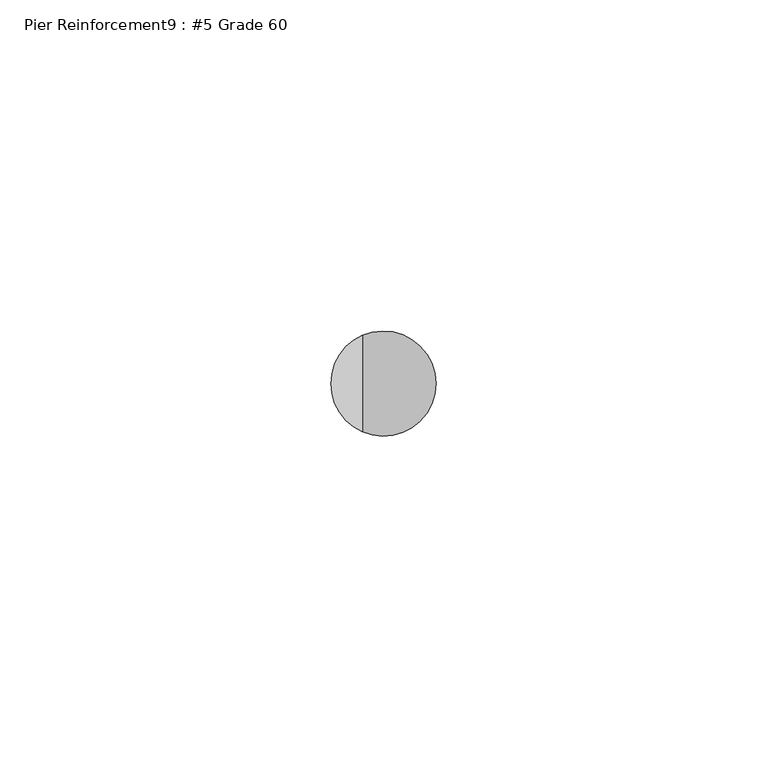
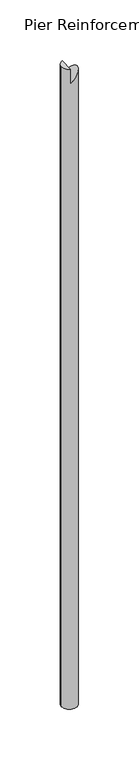
"""IFC4 building model written with IfcOpenShell, lengths in millimetres: proxy geometry, Pier Reinforcement9 : #5 Grade 60."""

from ifc_helpers import new_model, si_unit, frame, origin, place, context, project, spatial, circle_curve, ellipse_curve, source, transform, mapped, element, save
from ifc_brep_helpers import plane_surface, cylinder_surface, advanced_brep


def pier_reinforcement9_5_grade_60_f625620a(model_context):
    return source(origin(), model_context, "Body", "AdvancedBrep", [
        advanced_brep(
        [(590218.1172365, -534096.6663841, -47.625), (590222.8797365, -534103.941223, -47.625), (590222.8797365, -534089.3915452, -47.625), (590218.1172365, -534096.6663841, -733.425), (590233.9922365, -534096.6663841, -733.425), (590233.9922365, -534096.6663841, -52.3875), (590222.8797365, -534103.941223, -63.5), (590222.8797365, -534089.3915452, -63.5)],
        [
            (0, 1, circle_curve(frame((590226.0547365, -534096.6663841, -47.625), z_axis=(0.0, 0.0, 1.0), x_axis=(1.0, 0.0, 0.0)), 7.9375)),
            (1, 2),
            (2, 0, circle_curve(frame((590226.0547365, -534096.6663841, -47.625), z_axis=(0.0, 0.0, 1.0), x_axis=(1.0, 0.0, 0.0)), 7.9375)),
            (3, 4, circle_curve(frame((590226.0547365, -534096.6663841, -733.425), z_axis=(0.0, 0.0, -1.0), x_axis=(1.0, 0.0, 0.0)), 7.9375)),
            (4, 3, circle_curve(frame((590226.0547365, -534096.6663841, -733.425), z_axis=(0.0, 0.0, -1.0), x_axis=(1.0, 0.0, 0.0)), 7.9375)),
            (4, 5),
            (5, 6, ellipse_curve(frame((590226.0547365, -534096.6663841, -60.325), z_axis=(0.707106781186547, 0.0, -0.7071067811865481), x_axis=(0.7071067811865481, 0.0, 0.7071067811865468)), 11.2253202, 7.9375)),
            (6, 1),
            (0, 3),
            (2, 7),
            (7, 5, ellipse_curve(frame((590226.0547365, -534096.6663841, -60.325), z_axis=(0.707106781186547, 0.0, -0.7071067811865481), x_axis=(0.7071067811865481, 0.0, 0.7071067811865468)), 11.2253202, 7.9375)),
            (6, 7),
        ],
        [
            plane_surface(frame((590233.9922365, -534096.6663841, -47.625), z_axis=(0.0, 0.0, 1.0), x_axis=(0.0, 1.0, 0.0))),
            plane_surface(frame((590233.9922365, -534096.6663841, -733.425), z_axis=(0.0, 0.0, -1.0), x_axis=(0.0, -1.0, 0.0))),
            cylinder_surface(frame((590226.0547365, -534096.6663841, -733.425), z_axis=(0.0, 0.0, 1.0), x_axis=(1.0, 0.0, 0.0)), 7.9375),
            plane_surface(frame((590222.8797365, -534128.4163841, -47.625), z_axis=(1.0, 0.0, 0.0), x_axis=(0.0, 1.0, 0.0))),
            plane_surface(frame((590222.8797365, -534128.4163841, -63.5), z_axis=(-0.707106781186547, 0.0, 0.7071067811865481), x_axis=(0.0, 1.0, 0.0))),
        ],
        [
            (0, [[1, 2, 3]]),
            (1, [[4, 5]]),
            (2, [[-5, 6, 7, 8, -1, 9]]),
            (2, [[-4, -9, -3, 10, 11, -6]]),
            (3, [[12, -10, -2, -8]]),
            (4, [[-12, -7, -11]]),
        ],
    ),
    ])


if __name__ == "__main__":
    model = new_model("IFC4")
    model_context = context("Model", 3, world=origin())
    ifc_project = project(units=[si_unit("LENGTHUNIT", "METRE", prefix="MILLI")], contexts=[model_context])
    site = spatial("IfcSite", under=ifc_project)
    building = spatial("IfcBuilding", under=site)
    placement = place(None, origin())
    pier_reinforcement9_5_grade_60_shape = pier_reinforcement9_5_grade_60_f625620a(model_context)
    element("IfcBuildingElementProxy", 1, Name="Pier Reinforcement9 : #5 Grade 60", ObjectType="Pier Reinforcement9 : #5 Grade 60", at=placement, inside=building, context=model_context, shape_type="MappedRepresentation", body=[
        mapped(pier_reinforcement9_5_grade_60_shape, transform((0.0, 0.0, 0.0), x_axis=(1.0, 0.0, 0.0), y_axis=(0.0, 1.0, 0.0), z_axis=(0.0, 0.0, 1.0))),
    ])
    save(model, "model.ifc")

# Revit data of these elements
# Element 1 (IfcBuildingElementProxy, "Pier Reinforcement9 : #5 Grade 60")
#   Materials on its faces: "#4 GR. 60 REINF. @ 16\" O.C. EW."
# Materials
#   "#4 GR. 60 REINF. @ 16\" O.C. EW.": class "Generic", colour RGB 84 83 81, transparency 0, Cost = 0
